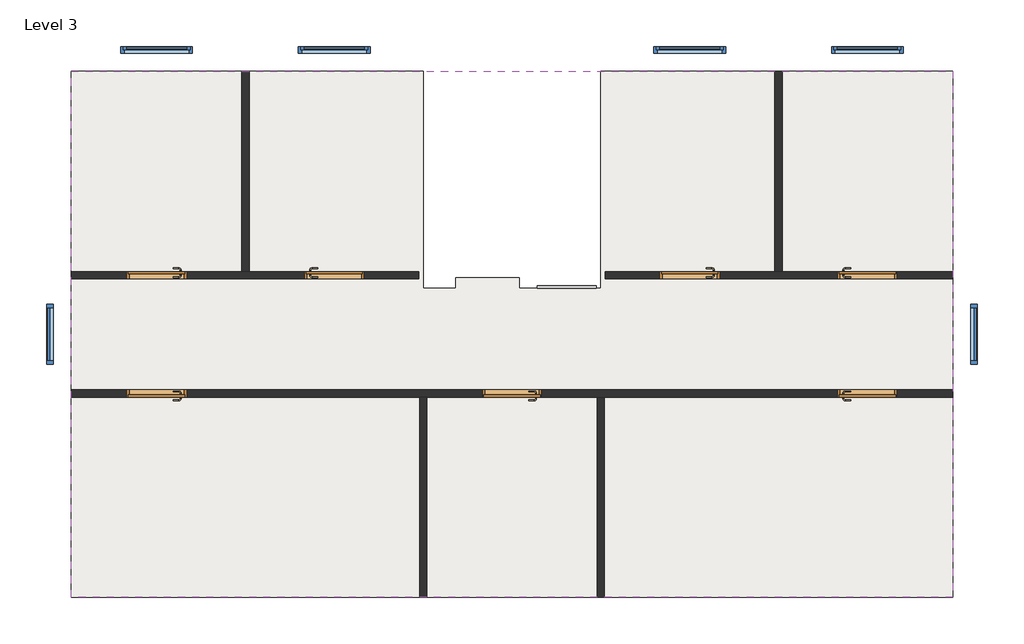
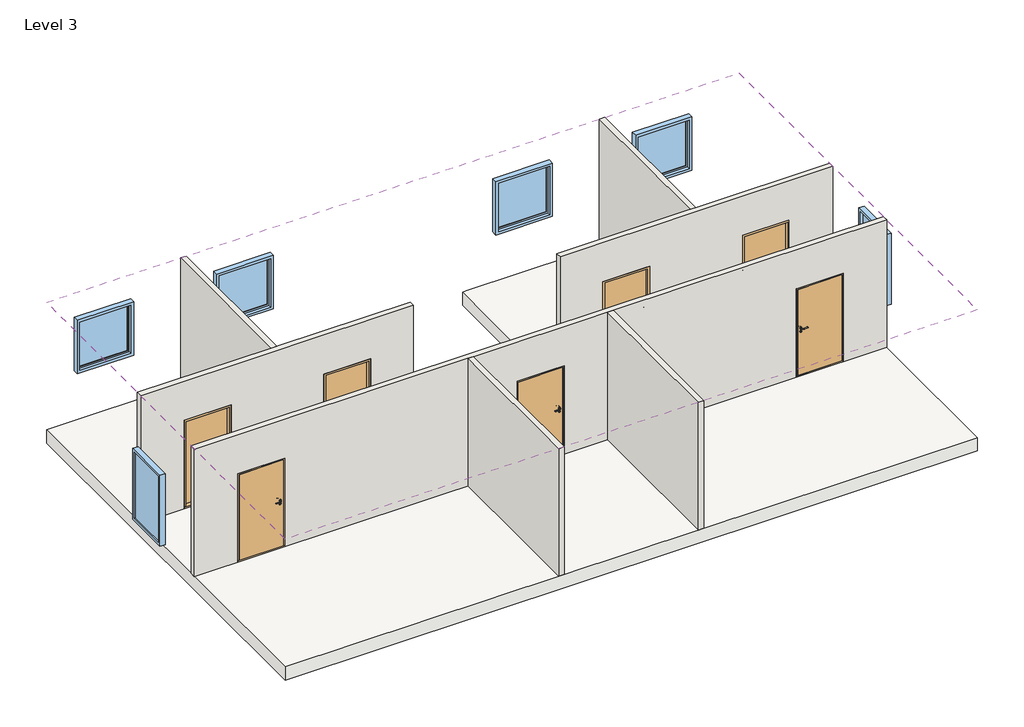
# One storey: 7 doors, 7 walls, 6 windows, 1 railing, 1 roof, 1 slab.
# Revit data of these elements (continued)
# Type "Single-Light : 12x12M" (continued)
#   Glass Thickness = 22 mm
#   Frame Width = 50 mm
#   Frame Depth = 50 mm
#   Exterior Direction [instance default] = 0.00°
#   Case Depth = 115 mm
#   Case Width = 45 mm
#   Default Sill Height = 800 mm
#   Width = 1188 mm
#   Sealing = no
#   Hinging = yes
#   Wall Closure = 1
#   Above Cutplane [instance default] = no
#   Wall Surface = none
#   Sill Plate = none
#   Glass = none
#   Frame/Mullion = none
#   Embrasure = none
#   Case/Transom = none
# Elements 1, 2, 3, 4, 5, 6, 7 (IfcDoor, "Int. Single-Flush : 10x20M")
#   Hinge Side = ""
#   Creator Organization = "© Danish Educational Content"
#   Creator Name = "© Erik Falck Jørgensen"
#   Creator Build = "2017.0801.0"
#   Interior Distance = 0 mm
#   Exterior Distance = 0 mm
#   Exterior Direction = 0.00°
#   Phase Created = New Construction
#   Materials on its faces: "Stainless Steel, Polished", "Default Frame/Mullion (Interior/Exterior)", "Default Door Panel (Exterior/Interior)"
# Element 8 (IfcRailing, "Sketch 1100mm")
#   Phase Created = New Construction
#   Materials on its faces: "Default Railings (Interior/Exterior)"
# Element 9 (IfcRoof, "Warm - 600mm Roofing Asphalt Filt / Concrete")
#   built-in parameter 1001705 = 32.4803 (stored number, unit not read)
#   built-in parameter 1001701 = -0.984252 (stored number, unit not read)
#   built-in parameter 1001710 = 33615
#   Phase Created = New Construction
#   Materials on its faces: "Concrete, Lightweight Precast", "Roofing Felt, Asphalt"
# Element 10 (IfcSlab, "Suspended - 300mm LW Concrete / Wood Planks")
#   built-in parameter 1001955 = 1.5708 (stored number, unit not read)
#   Height Offset From Level = 0 mm
#   Phase Created = New Construction
#   Materials on its faces: "Concrete, Lightweight Precast", "Wood Planks"
# Elements 11, 12, 13, 14 (IfcWall, "Interior - 120mm Drywall (25/70/25)")
#   Top Offset = 0 mm
#   Base Offset = 0 mm
#   wall height = 3200 mm
#   Phase Created = New Construction
#   Base Constraint = Level 3
#   Top Constraint = Roof
#   Materials on its faces: "Default Wall", "Gypsum Plasterboard"
# Elements 15, 16, 17 (IfcWall, "Interior - 120mm LW Concrete")
#   Top Offset = 0 mm
#   Base Offset = 0 mm
#   wall height = 3200 mm
#   Phase Created = New Construction
#   Base Constraint = Level 3
#   Top Constraint = Roof
#   Materials on its faces: "Concrete, Lightweight Precast"
# Element 18 (IfcWindow, "Fixed : 10x16M")
#   Mark = "26"
#   Creator Organization = "© Danish Educational Content"
#   Creator Name = "© Erik Falck Jørgensen"
#   Creator Build = "2017.0801.0"
#   Exterior Direction = 0.00°
#   Above Cutplane = no
#   Phase Created = New Construction
#   Materials on its faces: "Default Frame/Mullion (Interior/Exterior)", "Glass"
# Element 19 (IfcWindow, "Fixed : 10x16M")
#   Mark = "27"
#   Creator Organization = "© Danish Educational Content"
#   Creator Name = "© Erik Falck Jørgensen"
#   Creator Build = "2017.0801.0"
#   Exterior Direction = 0.00°
#   Above Cutplane = no
#   Phase Created = New Construction
#   Materials on its faces: "Default Frame/Mullion (Interior/Exterior)", "Glass"
# Element 20 (IfcWindow, "Single-Light : 12x12M")
#   Mark = "33"
#   Creator Organization = "© Danish Educational Content"
#   Creator Name = "© Erik Falck Jørgensen"
#   Creator Build = "2017.0801.0"
#   Exterior Direction = 0.00°
#   Above Cutplane = no
#   Phase Created = New Construction
#   Materials on its faces: "Default Frame/Mullion (Interior/Exterior)", "Glass"
# Element 21 (IfcWindow, "Single-Light : 12x12M")
#   Mark = "34"
#   Creator Organization = "© Danish Educational Content"
#   Creator Name = "© Erik Falck Jørgensen"
#   Creator Build = "2017.0801.0"
#   Exterior Direction = 0.00°
#   Above Cutplane = no
#   Phase Created = New Construction
#   Materials on its faces: "Default Frame/Mullion (Interior/Exterior)", "Glass"
# Element 22 (IfcWindow, "Single-Light : 12x12M")
#   Mark = "36"
#   Creator Organization = "© Danish Educational Content"
#   Creator Name = "© Erik Falck Jørgensen"
#   Creator Build = "2017.0801.0"
#   Exterior Direction = 0.00°
#   Above Cutplane = no
#   Phase Created = New Construction
#   Materials on its faces: "Default Frame/Mullion (Interior/Exterior)", "Glass"
# Element 23 (IfcWindow, "Single-Light : 12x12M")
#   Mark = "37"
#   Creator Organization = "© Danish Educational Content"
#   Creator Name = "© Erik Falck Jørgensen"
#   Creator Build = "2017.0801.0"
#   Exterior Direction = 0.00°
#   Above Cutplane = no
#   Phase Created = New Construction
#   Materials on its faces: "Default Frame/Mullion (Interior/Exterior)", "Glass"
# Materials
#   "Roofing Felt, Asphalt": class "Generic", colour RGB 30 30 30, transparency 0, Description = "Asfalt tagpap", Cost = 0
#   "Polystyrene": class "Insulation", colour RGB 255 240 100, transparency 0, Description = "Hård Polystyren", Cost = 0
#   "Concrete, Lightweight Precast": class "Concrete", colour RGB 180 180 180, transparency 0, Description = "Præfabrikeret letbeton", Cost = 0
#   "Wood Planks": class "Wood", colour RGB 117 91 64, transparency 0, Description = "Generisk trægulv", Cost = 0
#   "Flooring Underlay": class "Generic", colour RGB 255 0 0, transparency 0, Description = "Gulvunderlag", Cost = 0
#   "Concrete, Broom Finish": class "Concrete", colour RGB 80 80 80, transparency 0, Description = "Beton - afkostet overflade", Cost = 0
#   "Gypsum Plasterboard": class "Generic", colour RGB 180 180 180, transparency 0, Description = "Alm. indvendige gipsplader", Cost = 0
#   "Batt insulation": class "Insulation", colour RGB 255 240 100, transparency 0, Description = "Generisk blød isolering", Cost = 0
#   "Stainless Steel, Polished": class "Metal", colour RGB 180 180 180, transparency 0, Description = "Rustfri stål, poleret", Cost = 0
#   "Default Frame/Mullion (Interior/Exterior)": class "Generic", colour RGB 205 205 205, transparency 0, Description = "Udefineret karm/ramme materiale", Cost = 0
#   "Default Door Panel (Exterior/Interior)": class "Generic", colour RGB 205 205 205, transparency 0, Description = "Udefineret dørplade materiale", Cost = 0
#   "Default Railings (Interior/Exterior)": class "Generic", colour RGB 205 205 205, transparency 0, Description = "Udefineret gelænder materiale", Cost = 0
#   "Default Wall": class "Generic", colour RGB 180 180 180, transparency 0, Description = "Udefineret væg materiale", Cost = 0
#   "Glass": class "Glass", colour RGB 180 200 255, transparency 0.75, Description = "Generisk glas", Cost = 0
